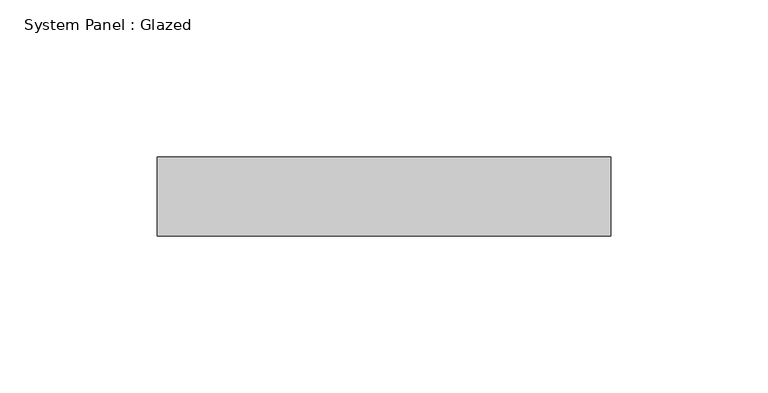
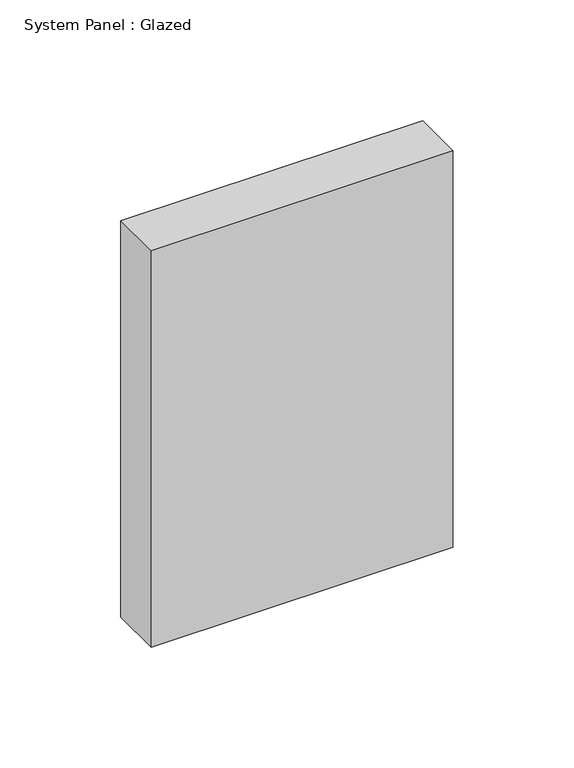
"""IFC4 building model written with IfcOpenShell, lengths in millimetres: plate geometry, System Panel : Glazed."""

from ifc_helpers import new_model, si_unit, origin, origin_with_axes, place, context, project, spatial, polyline, outline, extrude, source, transform, mapped, element, save


def system_panel_glazed_192fb397(model_context):
    return source(origin(), model_context, "Body", "SweptSolid", [
        extrude(outline(polyline([(72.019586, 24.5), (-72.019586, 24.5), (-72.019586, 49.5), (72.019586, 49.5), (72.019586, 24.5)])), origin_with_axes(), (0.0, 0.0, 1.0), 200.0),
    ])


if __name__ == "__main__":
    model = new_model("IFC4")
    model_context = context("Model", 3, world=origin())
    ifc_project = project(units=[si_unit("LENGTHUNIT", "METRE", prefix="MILLI")], contexts=[model_context])
    site = spatial("IfcSite", under=ifc_project)
    building = spatial("IfcBuilding", under=site)
    placement = place(None, origin())
    system_panel_glazed_shape = system_panel_glazed_192fb397(model_context)
    element("IfcPlate", 1, ObjectType="System Panel : Glazed", at=placement, inside=building, context=model_context, shape_type="MappedRepresentation", body=[
        mapped(system_panel_glazed_shape, transform((0.0, 0.0, 0.0), x_axis=(1.0, 0.0, 0.0), y_axis=(0.0, 1.0, 0.0), z_axis=(0.0, 0.0, 1.0))),
    ])
    save(model, "model.ifc")

# Revit data of these elements
# Element 1 (IfcPlate, "System Panel : Glazed")
#   Materials on its faces: "Glass"
# Materials
#   "Glass": class "Glass", colour RGB 218 227 224, transparency 0.85, Description = "Soda Lime Glass", Cost = 0
